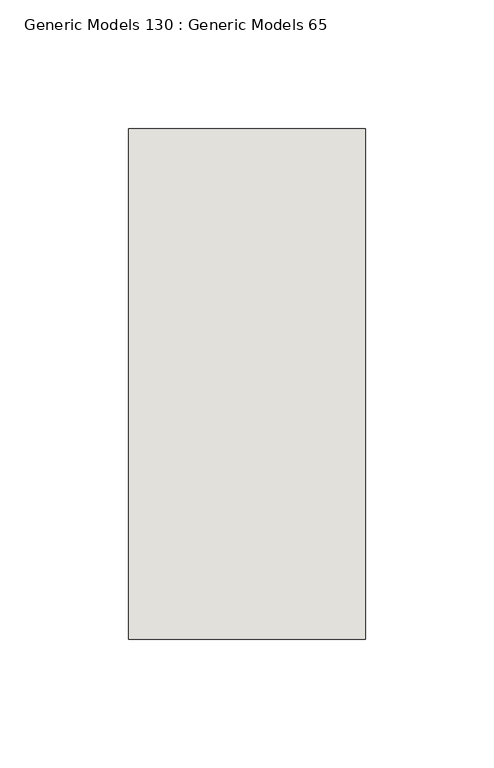
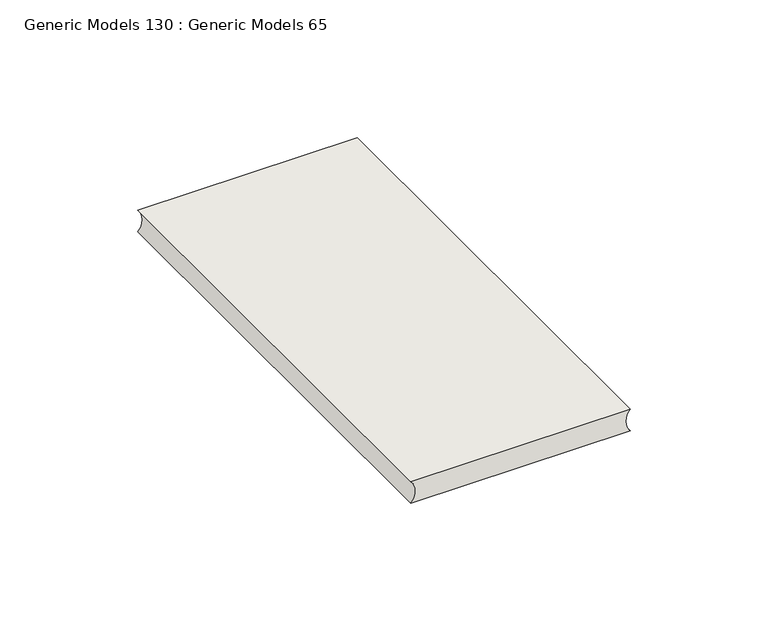
"""IFC4 building model written with IfcOpenShell, lengths in millimetres: wall geometry, Generic Models 130 : Generic Models 65."""

from ifc_helpers import new_model, si_unit, point, frame, frame_2d, origin, place, context, project, spatial, polyline, circle_curve, trimmed, segment, composite_curve, outline, extrude, source, transform, mapped, element, save


def generic_models_130_generic_models_65_b9b8dd6f(model_context):
    return source(origin(), model_context, "Body", "SweptSolid", [
        extrude(outline(composite_curve([segment(polyline([(1875.8712589, 375046.7901825), (1875.8712589, 374954.7151825)]), True, "CONTINUOUS"), segment(trimmed(circle_curve(frame_2d((1871.1087589, 374949.8321853)), 6.8209287), [point((1875.8712589, 374954.7151825))], [point((1866.3462589, 374954.7151825))], True, "CARTESIAN"), True, "CONTINUOUS"), segment(polyline([(1866.3462589, 374954.7151825), (1866.3462589, 375046.7901825)]), True, "CONTINUOUS"), segment(trimmed(circle_curve(frame_2d((1871.1087589, 375051.6731798)), 6.8209287), [point((1866.3462589, 375046.7901825))], [point((1875.8712589, 375046.7901825))], True, "CARTESIAN"), True, "CONTINUOUS")], self_intersect=False)), frame((0.0, 490.5375, 0.0), z_axis=(0.0, 1.0, 0.0), x_axis=(0.0, 0.0, 1.0)), (0.0, 0.0, 1.0), 198.4375),
    ])


if __name__ == "__main__":
    model = new_model("IFC4")
    model_context = context("Model", 3, world=origin())
    ifc_project = project(units=[si_unit("LENGTHUNIT", "METRE", prefix="MILLI")], contexts=[model_context])
    site = spatial("IfcSite", under=ifc_project)
    building = spatial("IfcBuilding", under=site)
    placement = place(None, origin())
    generic_models_130_generic_models_65_shape = generic_models_130_generic_models_65_b9b8dd6f(model_context)
    element("IfcWall", 1, ObjectType="Generic Models 130 : Generic Models 65", at=placement, inside=building, context=model_context, shape_type="MappedRepresentation", body=[
        mapped(generic_models_130_generic_models_65_shape, transform((0.0, 0.0, 0.0), x_axis=(1.0, 0.0, 0.0), y_axis=(0.0, 1.0, 0.0), z_axis=(0.0, 0.0, 1.0))),
    ])
    save(model, "model.ifc")

# Revit data of these elements
# Element 1 (IfcWall, "Generic Models 130 : Generic Models 65")
#   Materials on its faces: "MORTAR JOINT"
# Materials
#   "MORTAR JOINT": class "Generic", colour RGB 120 120 120, transparency 0, Cost = 0
